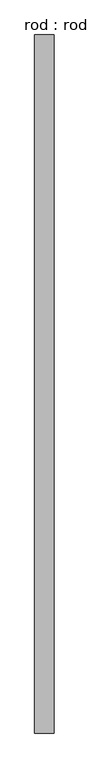
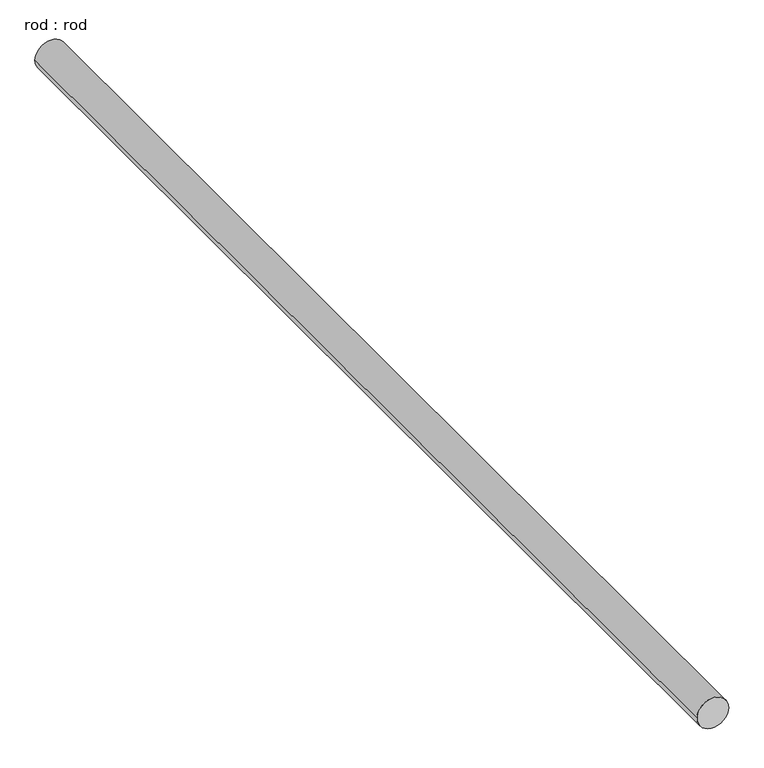
"""IFC4 building model written with IfcOpenShell, lengths in millimetres: proxy geometry, rod : rod."""

import ifcopenshell
import ifcopenshell.guid

model = None  # the IFC model being written
_history = None  # IfcOwnerHistory: only IFC2X3 demands one
_inside = {}  # id of a spatial element -> (the spatial element, [elements in it])
_under = {}  # id of a project, library or spatial element -> (it, [spatial elements below it])
_declared = {}  # id of a project -> (the project, [libraries it declares])
_typed = {}  # id of a type object -> (the type object, [elements of that type])
_made_of = {}  # id of a material, layer set ... -> (it, [elements and type objects made of it])


def new_model(schema):
    """Start an empty IFC model of exactly this schema.

    Asked for "IFC4X3", IfcOpenShell would pick the latest addendum, in which some entities
    have other attributes; the version numbers below select the first issue.
    IFC2X3 requires an IfcOwnerHistory on every rooted entity: one is made here for all.
    """
    global model, _history
    if schema == "IFC4X3":
        model = ifcopenshell.file(schema_version=(4, 3, 0, 0))
    else:
        model = ifcopenshell.file(schema=schema)
    _inside.clear()
    _under.clear()
    _declared.clear()
    _typed.clear()
    _made_of.clear()
    _history = None
    if model.schema == "IFC2X3":
        org = make("IfcOrganization", Name="unknown")
        user = make(
            "IfcPersonAndOrganization",
            ThePerson=make("IfcPerson", FamilyName="unknown"),
            TheOrganization=org,
        )
        app = make(
            "IfcApplication",
            ApplicationDeveloper=org,
            Version="unknown",
            ApplicationFullName="unknown",
            ApplicationIdentifier="unknown",
        )
        _history = make(
            "IfcOwnerHistory",
            OwningUser=user,
            OwningApplication=app,
            ChangeAction="ADDED",
            CreationDate=0,
        )
    return model


def make(cls, **values):
    """One entity of the class cls with the attributes given. An attribute that is None is left unset."""
    return model.create_entity(
        cls, **{name: value for name, value in values.items() if value is not None}
    )


def rooted(cls, **values):
    """An entity with a GlobalId (a new one), such as an element, a storey or a relation."""
    return make(cls, GlobalId=ifcopenshell.guid.new(), OwnerHistory=_history, **values)


def si_unit(unit_type, name, prefix=None):
    """IfcSIUnit, for example si_unit("LENGTHUNIT", "METRE", prefix="MILLI")."""
    return make("IfcSIUnit", UnitType=unit_type, Prefix=prefix, Name=name)


def assignment(units):
    """IfcUnitAssignment: the units of a project."""
    return None if units is None else make("IfcUnitAssignment", Units=units)


def point(xyz):
    """IfcCartesianPoint."""
    return None if xyz is None else make("IfcCartesianPoint", Coordinates=xyz)


def direction(xyz):
    """IfcDirection."""
    return None if xyz is None else make("IfcDirection", DirectionRatios=xyz)


def frame(location, z_axis=None, x_axis=None):
    """IfcAxis2Placement3D, a coordinate frame: its origin and axes. An axis left out is left unset."""
    return make(
        "IfcAxis2Placement3D",
        Location=point(location),
        Axis=direction(z_axis),
        RefDirection=direction(x_axis),
    )


def frame_2d(location, x_axis=None):
    """IfcAxis2Placement2D, a coordinate frame in the plane: its origin and x axis."""
    return make(
        "IfcAxis2Placement2D", Location=point(location), RefDirection=direction(x_axis)
    )


def origin():
    """The frame at (0, 0, 0) with its axes left unset."""
    return frame((0.0, 0.0, 0.0))


def place(relative_to, where):
    """IfcLocalPlacement: puts the frame where relative to a parent placement (None: the world)."""
    return make(
        "IfcLocalPlacement", PlacementRelTo=relative_to, RelativePlacement=where
    )


def context(
    kind, dimensions, precision=None, world=None, true_north=None, identifier=None
):
    """IfcGeometricRepresentationContext, for example the 3D "Model" context."""
    return make(
        "IfcGeometricRepresentationContext",
        ContextIdentifier=identifier,
        ContextType=kind,
        CoordinateSpaceDimension=dimensions,
        Precision=precision,
        WorldCoordinateSystem=world,
        TrueNorth=true_north,
    )


def project(units=None, contexts=None):
    """IfcProject with its units and contexts."""
    return rooted(
        "IfcProject",
        Name="project",
        RepresentationContexts=contexts,
        UnitsInContext=assignment(units),
    )


def spatial(cls, under=None, at=None, **own):
    """A site, building, storey or space (cls), placed at a placement, below another one or the project."""
    s = rooted(cls, ObjectPlacement=at, **own)
    if under is not None:
        _under.setdefault(under.id(), (under, []))[1].append(s)
    return s


def circle_curve(where, radius):
    """IfcCircle in the frame where."""
    return make("IfcCircle", Position=where, Radius=radius)


def trimmed(basis, trim1, trim2, sense, master):
    """IfcTrimmedCurve: the piece of a basis curve between two trims."""
    return make(
        "IfcTrimmedCurve",
        BasisCurve=basis,
        Trim1=trim1,
        Trim2=trim2,
        SenseAgreement=sense,
        MasterRepresentation=master,
    )


def segment(curve, same_sense, transition):
    """IfcCompositeCurveSegment."""
    return make(
        "IfcCompositeCurveSegment",
        Transition=transition,
        SameSense=same_sense,
        ParentCurve=curve,
    )


def composite_curve(segments, self_intersect=None):
    """IfcCompositeCurve: segments joined end to end."""
    return make("IfcCompositeCurve", Segments=segments, SelfIntersect=self_intersect)


def outline(outer, holes=None, kind="AREA"):
    """IfcArbitraryClosedProfileDef: a profile drawn as a closed curve; with holes, ...WithVoids."""
    if holes is None:
        return make("IfcArbitraryClosedProfileDef", ProfileType=kind, OuterCurve=outer)
    return make(
        "IfcArbitraryProfileDefWithVoids",
        ProfileType=kind,
        OuterCurve=outer,
        InnerCurves=holes,
    )


def extrude(swept, where, along, depth):
    """IfcExtrudedAreaSolid: the profile swept, set in the frame where, extruded along a direction by depth."""
    return make(
        "IfcExtrudedAreaSolid",
        SweptArea=swept,
        Position=where,
        ExtrudedDirection=direction(along),
        Depth=depth,
    )


def shape(context_of_items, identifier, shape_type, items):
    """IfcShapeRepresentation: the items that make up one representation, for example the "Body"."""
    return make(
        "IfcShapeRepresentation",
        ContextOfItems=context_of_items,
        RepresentationIdentifier=identifier,
        RepresentationType=shape_type,
        Items=items,
    )


def source(mapping_origin, context_of_items, identifier, shape_type, items):
    """IfcRepresentationMap: a shape defined once, which mapped items show again and again."""
    return make(
        "IfcRepresentationMap",
        MappingOrigin=mapping_origin,
        MappedRepresentation=shape(context_of_items, identifier, shape_type, items),
    )


def transform(
    local_origin,
    x_axis=None,
    y_axis=None,
    z_axis=None,
    scale=None,
    scale2=None,
    scale3=None,
    uniform=True,
):
    """IfcCartesianTransformationOperator3D, or its non-uniform kind. x_axis, y_axis, z_axis: its Axis1, 2, 3."""
    if uniform:
        return make(
            "IfcCartesianTransformationOperator3D",
            Axis1=direction(x_axis),
            Axis2=direction(y_axis),
            LocalOrigin=point(local_origin),
            Scale=scale,
            Axis3=direction(z_axis),
        )
    return make(
        "IfcCartesianTransformationOperator3DnonUniform",
        Axis1=direction(x_axis),
        Axis2=direction(y_axis),
        LocalOrigin=point(local_origin),
        Scale=scale,
        Axis3=direction(z_axis),
        Scale2=scale2,
        Scale3=scale3,
    )


def mapped(mapping_source, mapping_target):
    """IfcMappedItem: shows the shape of a source again, moved by a transform."""
    return make(
        "IfcMappedItem", MappingSource=mapping_source, MappingTarget=mapping_target
    )


def made_of(thing, what):
    """Note that an element or type object is made of a material, layer set ...; save() writes the relation."""
    if what is not None:
        _made_of.setdefault(what.id(), (what, []))[1].append(thing)
    return thing


def element(
    cls,
    number,
    at=None,
    inside=None,
    cuts=None,
    type_object=None,
    material=None,
    context=None,
    identifier="Body",
    shape_type=None,
    held_by="IfcProductDefinitionShape",
    body=None,
    shapes=None,
    **own,
):
    """One element of the class cls, such as IfcWall. Its Tag is "e" and its number.

    at: its placement. inside: the storey or other place that contains it. cuts: it is an
    opening in that element (IfcRelVoidsElement). A single representation is given by context,
    identifier, shape_type and body (its items); several are given by shapes. held_by: the class
    of the entity that holds the representations. save() writes the other relations.
    """
    e = rooted(cls, Tag="e%d" % number, ObjectPlacement=at, **own)
    if body is not None:
        shapes = [shape(context, identifier, shape_type, body)]
    if shapes is not None:
        e.Representation = make(held_by, Representations=shapes)
    if inside is not None:
        _inside.setdefault(inside.id(), (inside, []))[1].append(e)
    if cuts is not None:
        rooted(
            "IfcRelVoidsElement", RelatingBuildingElement=cuts, RelatedOpeningElement=e
        )
    if type_object is not None:
        _typed.setdefault(type_object.id(), (type_object, []))[1].append(e)
    return made_of(e, material)


def aggregate(whole, parts):
    """IfcRelAggregates: a whole, such as a stair, and the parts it consists of."""
    return rooted("IfcRelAggregates", RelatingObject=whole, RelatedObjects=parts)


def save(model, path):
    """Write the relations noted so far, then the file.

    IfcRelAggregates (storeys below a building ...), IfcRelContainedInSpatialStructure (elements
    in a storey), IfcRelDefinesByType, IfcRelAssociatesMaterial and IfcRelDeclares: one each for
    every whole, place, type object, material and project.
    """
    for whole, parts in _under.values():
        aggregate(whole, parts)
    for where, things in _inside.values():
        rooted(
            "IfcRelContainedInSpatialStructure",
            RelatedElements=things,
            RelatingStructure=where,
        )
    for kind, things in _typed.values():
        rooted("IfcRelDefinesByType", RelatedObjects=things, RelatingType=kind)
    for what, things in _made_of.values():
        rooted("IfcRelAssociatesMaterial", RelatedObjects=things, RelatingMaterial=what)
    for by, libraries in _declared.values():
        rooted("IfcRelDeclares", RelatingContext=by, RelatedDefinitions=libraries)
    model.write(path)


def rod_rod_c933ca01(model_context):
    return source(origin(), model_context, "Body", "SweptSolid", [
        extrude(outline(composite_curve([segment(trimmed(circle_curve(frame_2d((0.0108462, 0.0)), 200.0), [point((0.0108462, 200.0))], [point((0.0108462, -200.0))], False, "CARTESIAN"), True, "CONTINUOUS"), segment(trimmed(circle_curve(frame_2d((0.0108462, 0.0)), 200.0), [point((0.0108462, -200.0))], [point((0.0108462, 200.0))], False, "CARTESIAN"), True, "CONTINUOUS")], self_intersect=False)), frame((0.0, -3154.0504105, 0.0), z_axis=(0.0, 1.0, 0.0), x_axis=(0.0, 0.0, 1.0)), (0.0, 0.0, 1.0), 14493.5580518),
    ])


if __name__ == "__main__":
    model = new_model("IFC4")
    model_context = context("Model", 3, world=origin())
    ifc_project = project(units=[si_unit("LENGTHUNIT", "METRE", prefix="MILLI")], contexts=[model_context])
    site = spatial("IfcSite", under=ifc_project)
    building = spatial("IfcBuilding", under=site)
    placement = place(None, origin())
    rod_rod_shape = rod_rod_c933ca01(model_context)
    element("IfcBuildingElementProxy", 1, Name="rod : rod", ObjectType="rod : rod", at=placement, inside=building, context=model_context, shape_type="MappedRepresentation", body=[
        mapped(rod_rod_shape, transform((0.0, 0.0, 0.0), x_axis=(1.0, 0.0, 0.0), y_axis=(0.0, 1.0, 0.0), z_axis=(0.0, 0.0, 1.0))),
    ])
    save(model, "model.ifc")

# Revit data of these elements
# Type "rod : rod"
#   Default Elevation = 0
